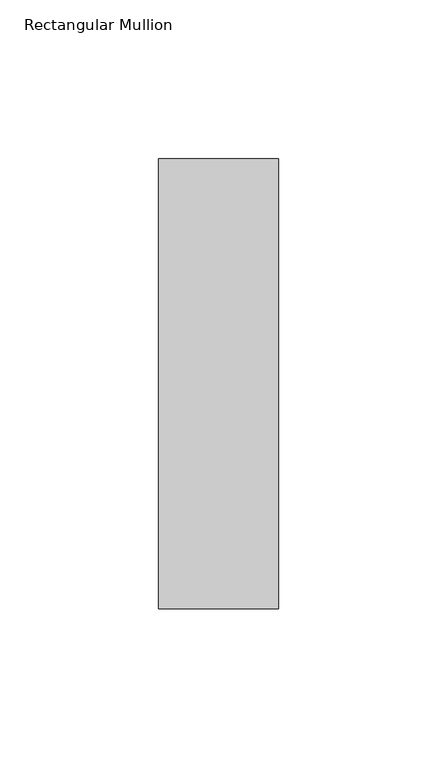
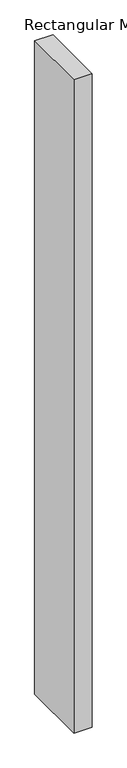
"""IFC4 building model written with IfcOpenShell, lengths in millimetres: member geometry, Rectangular Mullion : NLRS_21_CWM_hsb-regel 38x142_gen_rsf."""

from ifc_helpers import new_model, si_unit, frame, origin, place, context, project, spatial, polyline, outline, extrude, source, transform, mapped, element, save


def rectangular_mullion_de1563bf(model_context):
    return source(origin(), model_context, "Body", "SweptSolid", [
        extrude(outline(polyline([(0.0, -71.0), (-38.0, -71.0), (-38.0, 71.0), (0.0, 71.0), (0.0, -71.0)])), frame((0.0, 0.0, -1440.0), z_axis=(0.0, 0.0, 1.0), x_axis=(1.0, 0.0, 0.0)), (0.0, 0.0, 1.0), 1440.0),
    ])


if __name__ == "__main__":
    model = new_model("IFC4")
    model_context = context("Model", 3, world=origin())
    ifc_project = project(units=[si_unit("LENGTHUNIT", "METRE", prefix="MILLI")], contexts=[model_context])
    site = spatial("IfcSite", under=ifc_project)
    building = spatial("IfcBuilding", under=site)
    placement = place(None, origin())
    rectangular_mullion_shape = rectangular_mullion_de1563bf(model_context)
    element("IfcMember", 1, ObjectType="Rectangular Mullion : NLRS_21_CWM_hsb-regel 38x142_gen_rsf", at=placement, inside=building, context=model_context, shape_type="MappedRepresentation", body=[
        mapped(rectangular_mullion_shape, transform((0.0, 0.0, 0.0), x_axis=(1.0, 0.0, 0.0), y_axis=(0.0, 1.0, 0.0), z_axis=(0.0, 0.0, 1.0))),
    ])
    save(model, "model.ifc")

# Revit data of these elements
# Type "Rectangular Mullion : NLRS_21_CWM_hsb-regel 38x142_gen_rsf"
#   Export Type to IFC As = "IfcWall"
#   Type IfcGUID = "07M7mRoiH1CR8m_RSKIwpF"
#   Assembly Code = "21.10"
#   built-in parameter 1007322 = 0.465879 (stored number, unit not read)
#   built-in parameter 1007321 = 0.062336 (stored number, unit not read)
#   built-in parameter 1007320 = 0.062336 (stored number, unit not read)
# Element 1 (IfcMember, "Rectangular Mullion : NLRS_21_CWM_hsb-regel 38x142_gen_rsf")
#   Materials on its faces: "NLRS_i2_hout naaldhout vuren_gen_rsf"
# Materials
#   "NLRS_i2_hout naaldhout vuren_gen_rsf": class "I - Hout", colour RGB 234 199 147, transparency 0, Keynote = "i2", Manufacturer = "Revit Standards Foundation", URL = "www.revitstandards.org", Description = "hout vuren", Cost = 0
